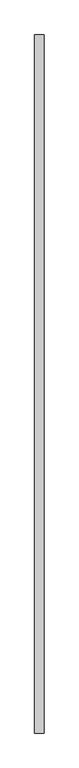
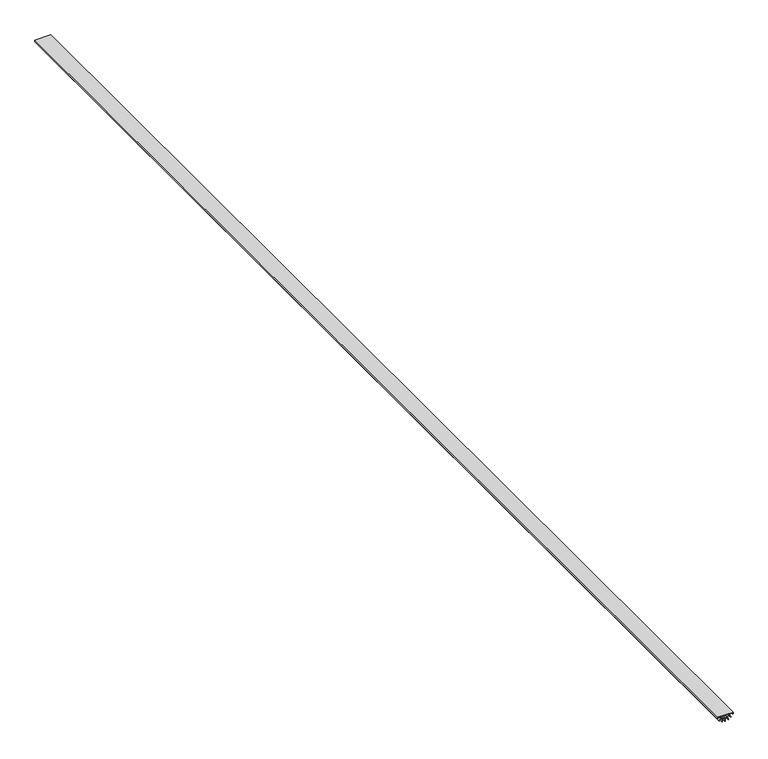
"""IFC4 building model written with IfcOpenShell, lengths in millimetres: proxy geometry, Door frame15:Door frame014:296522 : Door frame15:Door frame014:296522."""

from ifc_helpers import new_model, si_unit, frame, origin, place, context, project, spatial, polyline, outline, extrude, source, transform, mapped, element, save


def generic_models_b09664a4(model_context):
    return source(origin(), model_context, "Body", "SweptSolid", [
        extrude(outline(polyline([(36583.8229098, 20301.8801325), (36578.3756733, 20301.8801325), (36578.3756733, 20302.6738825), (36583.8229098, 20302.6738825), (36584.304169, 20305.4285942), (36579.1830903, 20307.2925032), (36579.4545674, 20308.0383848), (36584.573299, 20306.17533), (36585.9800182, 20308.6296562), (36581.8052868, 20312.1326937), (36582.3155014, 20312.7407399), (36586.4883159, 20309.2393109), (36588.5541303, 20311.0032398), (36588.5541303, 20313.9953987), (36587.284361, 20313.9953987), (36587.284361, 20315.6939695), (36589.8546103, 20315.6939695), (36589.8546103, 20288.5520522), (36587.284361, 20288.5520522), (36587.284361, 20290.5586163), (36588.5541303, 20290.5586163), (36588.5541303, 20293.5507752), (36586.5323252, 20295.2661451), (36582.3575787, 20291.7631274), (36581.8473669, 20292.371176), (36586.0201974, 20295.8725859), (36584.5980367, 20298.3180251), (36579.4769756, 20296.4540782), (36579.2054928, 20297.1999576), (36584.3242102, 20299.0630515), (36583.8229098, 20301.8801325)]), holes=[polyline([(36588.5541303, 20294.6590116), (36588.5541303, 20309.8950034), (36586.6136518, 20307.8829204), (36585.2069325, 20305.4285942), (36584.7256733, 20302.6738825), (36584.7256733, 20301.8801325), (36585.2269736, 20299.0630515), (36586.6491343, 20296.6176123), (36588.5541303, 20294.6590116)])]), frame((0.0, -774.5581156, 0.0), z_axis=(0.0, 1.0, 0.0), x_axis=(0.0, 0.0, 1.0)), (0.0, 0.0, 1.0), 1999.85),
    ])


if __name__ == "__main__":
    model = new_model("IFC4")
    model_context = context("Model", 3, world=origin())
    ifc_project = project(units=[si_unit("LENGTHUNIT", "METRE", prefix="MILLI")], contexts=[model_context])
    site = spatial("IfcSite", under=ifc_project)
    building = spatial("IfcBuilding", under=site)
    placement = place(None, origin())
    generic_models_shape = generic_models_b09664a4(model_context)
    element("IfcBuildingElementProxy", 1, Name="Door frame15:Door frame014:296522 : Door frame15:Door frame014:296522", ObjectType="Door frame15:Door frame014:296522 : Door frame15:Door frame014:296522", at=placement, inside=building, context=model_context, shape_type="MappedRepresentation", body=[
        mapped(generic_models_shape, transform((0.0, 0.0, 0.0), x_axis=(1.0, 0.0, 0.0), y_axis=(0.0, 1.0, 0.0), z_axis=(0.0, 0.0, 1.0))),
    ])
    save(model, "model.ifc")

# Revit data of these elements
# Type "Door frame15:Door frame014:296522 : Door frame15:Door frame014:296522"
#   NameOverride = "Door frame15:Door frame014:296522"
#   ObjectTypeOverride = "Door frame15:Door frame014"
#   Reference = "Door frame014"
#   Category = "Generic Models"
#   Tag = "296522"
# Element 1 (IfcBuildingElementProxy, "Door frame15:Door frame014:296522 : Door frame15:Door frame014:296522")
#   Materials on its faces: "WEATHERSTRIPPING SWEEP 171983"
# Materials
#   "WEATHERSTRIPPING SWEEP 171983": class "Unassigned", colour RGB 212 179 113, transparency 0
